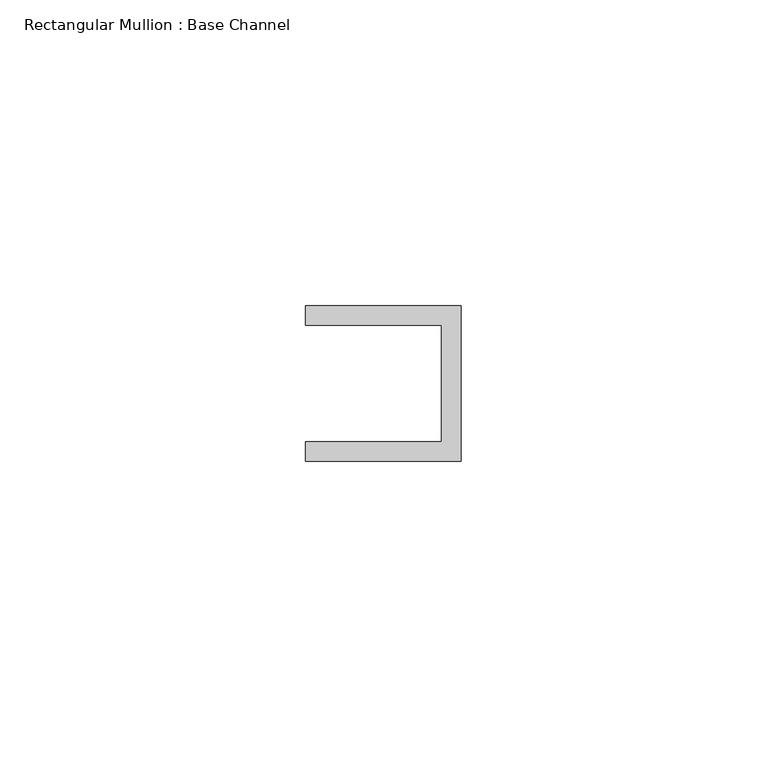
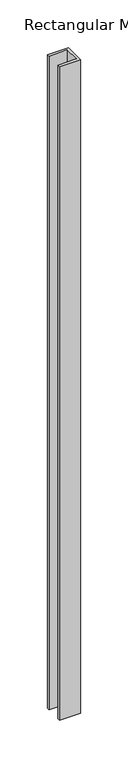
"""IFC4 building model written with IfcOpenShell, lengths in millimetres: member geometry, Rectangular Mullion : Base Channel."""

import ifcopenshell
import ifcopenshell.guid

model = None  # the IFC model being written
_history = None  # IfcOwnerHistory: only IFC2X3 demands one
_inside = {}  # id of a spatial element -> (the spatial element, [elements in it])
_under = {}  # id of a project, library or spatial element -> (it, [spatial elements below it])
_declared = {}  # id of a project -> (the project, [libraries it declares])
_typed = {}  # id of a type object -> (the type object, [elements of that type])
_made_of = {}  # id of a material, layer set ... -> (it, [elements and type objects made of it])


def new_model(schema):
    """Start an empty IFC model of exactly this schema.

    Asked for "IFC4X3", IfcOpenShell would pick the latest addendum, in which some entities
    have other attributes; the version numbers below select the first issue.
    IFC2X3 requires an IfcOwnerHistory on every rooted entity: one is made here for all.
    """
    global model, _history
    if schema == "IFC4X3":
        model = ifcopenshell.file(schema_version=(4, 3, 0, 0))
    else:
        model = ifcopenshell.file(schema=schema)
    _inside.clear()
    _under.clear()
    _declared.clear()
    _typed.clear()
    _made_of.clear()
    _history = None
    if model.schema == "IFC2X3":
        org = make("IfcOrganization", Name="unknown")
        user = make(
            "IfcPersonAndOrganization",
            ThePerson=make("IfcPerson", FamilyName="unknown"),
            TheOrganization=org,
        )
        app = make(
            "IfcApplication",
            ApplicationDeveloper=org,
            Version="unknown",
            ApplicationFullName="unknown",
            ApplicationIdentifier="unknown",
        )
        _history = make(
            "IfcOwnerHistory",
            OwningUser=user,
            OwningApplication=app,
            ChangeAction="ADDED",
            CreationDate=0,
        )
    return model


def make(cls, **values):
    """One entity of the class cls with the attributes given. An attribute that is None is left unset."""
    return model.create_entity(
        cls, **{name: value for name, value in values.items() if value is not None}
    )


def rooted(cls, **values):
    """An entity with a GlobalId (a new one), such as an element, a storey or a relation."""
    return make(cls, GlobalId=ifcopenshell.guid.new(), OwnerHistory=_history, **values)


def si_unit(unit_type, name, prefix=None):
    """IfcSIUnit, for example si_unit("LENGTHUNIT", "METRE", prefix="MILLI")."""
    return make("IfcSIUnit", UnitType=unit_type, Prefix=prefix, Name=name)


def assignment(units):
    """IfcUnitAssignment: the units of a project."""
    return None if units is None else make("IfcUnitAssignment", Units=units)


def point(xyz):
    """IfcCartesianPoint."""
    return None if xyz is None else make("IfcCartesianPoint", Coordinates=xyz)


def direction(xyz):
    """IfcDirection."""
    return None if xyz is None else make("IfcDirection", DirectionRatios=xyz)


def frame(location, z_axis=None, x_axis=None):
    """IfcAxis2Placement3D, a coordinate frame: its origin and axes. An axis left out is left unset."""
    return make(
        "IfcAxis2Placement3D",
        Location=point(location),
        Axis=direction(z_axis),
        RefDirection=direction(x_axis),
    )


def origin():
    """The frame at (0, 0, 0) with its axes left unset."""
    return frame((0.0, 0.0, 0.0))


def place(relative_to, where):
    """IfcLocalPlacement: puts the frame where relative to a parent placement (None: the world)."""
    return make(
        "IfcLocalPlacement", PlacementRelTo=relative_to, RelativePlacement=where
    )


def context(
    kind, dimensions, precision=None, world=None, true_north=None, identifier=None
):
    """IfcGeometricRepresentationContext, for example the 3D "Model" context."""
    return make(
        "IfcGeometricRepresentationContext",
        ContextIdentifier=identifier,
        ContextType=kind,
        CoordinateSpaceDimension=dimensions,
        Precision=precision,
        WorldCoordinateSystem=world,
        TrueNorth=true_north,
    )


def project(units=None, contexts=None):
    """IfcProject with its units and contexts."""
    return rooted(
        "IfcProject",
        Name="project",
        RepresentationContexts=contexts,
        UnitsInContext=assignment(units),
    )


def spatial(cls, under=None, at=None, **own):
    """A site, building, storey or space (cls), placed at a placement, below another one or the project."""
    s = rooted(cls, ObjectPlacement=at, **own)
    if under is not None:
        _under.setdefault(under.id(), (under, []))[1].append(s)
    return s


def polyline(points):
    """IfcPolyline through the points."""
    return make("IfcPolyline", Points=[point(p) for p in points])


def outline(outer, holes=None, kind="AREA"):
    """IfcArbitraryClosedProfileDef: a profile drawn as a closed curve; with holes, ...WithVoids."""
    if holes is None:
        return make("IfcArbitraryClosedProfileDef", ProfileType=kind, OuterCurve=outer)
    return make(
        "IfcArbitraryProfileDefWithVoids",
        ProfileType=kind,
        OuterCurve=outer,
        InnerCurves=holes,
    )


def extrude(swept, where, along, depth):
    """IfcExtrudedAreaSolid: the profile swept, set in the frame where, extruded along a direction by depth."""
    return make(
        "IfcExtrudedAreaSolid",
        SweptArea=swept,
        Position=where,
        ExtrudedDirection=direction(along),
        Depth=depth,
    )


def shape(context_of_items, identifier, shape_type, items):
    """IfcShapeRepresentation: the items that make up one representation, for example the "Body"."""
    return make(
        "IfcShapeRepresentation",
        ContextOfItems=context_of_items,
        RepresentationIdentifier=identifier,
        RepresentationType=shape_type,
        Items=items,
    )


def source(mapping_origin, context_of_items, identifier, shape_type, items):
    """IfcRepresentationMap: a shape defined once, which mapped items show again and again."""
    return make(
        "IfcRepresentationMap",
        MappingOrigin=mapping_origin,
        MappedRepresentation=shape(context_of_items, identifier, shape_type, items),
    )


def transform(
    local_origin,
    x_axis=None,
    y_axis=None,
    z_axis=None,
    scale=None,
    scale2=None,
    scale3=None,
    uniform=True,
):
    """IfcCartesianTransformationOperator3D, or its non-uniform kind. x_axis, y_axis, z_axis: its Axis1, 2, 3."""
    if uniform:
        return make(
            "IfcCartesianTransformationOperator3D",
            Axis1=direction(x_axis),
            Axis2=direction(y_axis),
            LocalOrigin=point(local_origin),
            Scale=scale,
            Axis3=direction(z_axis),
        )
    return make(
        "IfcCartesianTransformationOperator3DnonUniform",
        Axis1=direction(x_axis),
        Axis2=direction(y_axis),
        LocalOrigin=point(local_origin),
        Scale=scale,
        Axis3=direction(z_axis),
        Scale2=scale2,
        Scale3=scale3,
    )


def mapped(mapping_source, mapping_target):
    """IfcMappedItem: shows the shape of a source again, moved by a transform."""
    return make(
        "IfcMappedItem", MappingSource=mapping_source, MappingTarget=mapping_target
    )


def made_of(thing, what):
    """Note that an element or type object is made of a material, layer set ...; save() writes the relation."""
    if what is not None:
        _made_of.setdefault(what.id(), (what, []))[1].append(thing)
    return thing


def element(
    cls,
    number,
    at=None,
    inside=None,
    cuts=None,
    type_object=None,
    material=None,
    context=None,
    identifier="Body",
    shape_type=None,
    held_by="IfcProductDefinitionShape",
    body=None,
    shapes=None,
    **own,
):
    """One element of the class cls, such as IfcWall. Its Tag is "e" and its number.

    at: its placement. inside: the storey or other place that contains it. cuts: it is an
    opening in that element (IfcRelVoidsElement). A single representation is given by context,
    identifier, shape_type and body (its items); several are given by shapes. held_by: the class
    of the entity that holds the representations. save() writes the other relations.
    """
    e = rooted(cls, Tag="e%d" % number, ObjectPlacement=at, **own)
    if body is not None:
        shapes = [shape(context, identifier, shape_type, body)]
    if shapes is not None:
        e.Representation = make(held_by, Representations=shapes)
    if inside is not None:
        _inside.setdefault(inside.id(), (inside, []))[1].append(e)
    if cuts is not None:
        rooted(
            "IfcRelVoidsElement", RelatingBuildingElement=cuts, RelatedOpeningElement=e
        )
    if type_object is not None:
        _typed.setdefault(type_object.id(), (type_object, []))[1].append(e)
    return made_of(e, material)


def aggregate(whole, parts):
    """IfcRelAggregates: a whole, such as a stair, and the parts it consists of."""
    return rooted("IfcRelAggregates", RelatingObject=whole, RelatedObjects=parts)


def save(model, path):
    """Write the relations noted so far, then the file.

    IfcRelAggregates (storeys below a building ...), IfcRelContainedInSpatialStructure (elements
    in a storey), IfcRelDefinesByType, IfcRelAssociatesMaterial and IfcRelDeclares: one each for
    every whole, place, type object, material and project.
    """
    for whole, parts in _under.values():
        aggregate(whole, parts)
    for where, things in _inside.values():
        rooted(
            "IfcRelContainedInSpatialStructure",
            RelatedElements=things,
            RelatingStructure=where,
        )
    for kind, things in _typed.values():
        rooted("IfcRelDefinesByType", RelatedObjects=things, RelatingType=kind)
    for what, things in _made_of.values():
        rooted("IfcRelAssociatesMaterial", RelatedObjects=things, RelatingMaterial=what)
    for by, libraries in _declared.values():
        rooted("IfcRelDeclares", RelatingContext=by, RelatedDefinitions=libraries)
    model.write(path)


def rectangular_mullion_base_channel_13c842bd(model_context):
    return source(origin(), model_context, "Body", "SweptSolid", [
        extrude(outline(polyline([(0.0, -12.7), (-25.4, -12.7), (-25.4, -9.525), (-3.175, -9.525), (-3.175, 9.525), (-25.4, 9.525), (-25.4, 12.7), (0.0, 12.7), (0.0, -12.7)])), frame((0.0, 0.0, -838.1999999), z_axis=(0.0, 0.0, 1.0), x_axis=(1.0, 0.0, 0.0)), (0.0, 0.0, 1.0), 838.1999999),
    ])


if __name__ == "__main__":
    model = new_model("IFC4")
    model_context = context("Model", 3, world=origin())
    ifc_project = project(units=[si_unit("LENGTHUNIT", "METRE", prefix="MILLI")], contexts=[model_context])
    site = spatial("IfcSite", under=ifc_project)
    building = spatial("IfcBuilding", under=site)
    placement = place(None, origin())
    rectangular_mullion_base_channel_shape = rectangular_mullion_base_channel_13c842bd(model_context)
    element("IfcMember", 1, ObjectType="Rectangular Mullion : Base Channel", at=placement, inside=building, context=model_context, shape_type="MappedRepresentation", body=[
        mapped(rectangular_mullion_base_channel_shape, transform((0.0, 0.0, 0.0), x_axis=(1.0, 0.0, 0.0), y_axis=(0.0, 1.0, 0.0), z_axis=(0.0, 0.0, 1.0))),
    ])
    save(model, "model.ifc")

# Revit data of these elements
# Type "Rectangular Mullion : Base Channel"
#   built-in parameter 1007322 = 0.0833333 (stored number, unit not read)
#   built-in parameter 1007321 = 0.0416667 (stored number, unit not read)
#   built-in parameter 1007320 = -0.03125 (stored number, unit not read)
# Element 1 (IfcMember, "Rectangular Mullion : Base Channel")
#   Materials on its faces: "ALUM"
# Materials
#   "ALUM": class "Generic", colour RGB 157 157 157, transparency 0, Cost = 0
